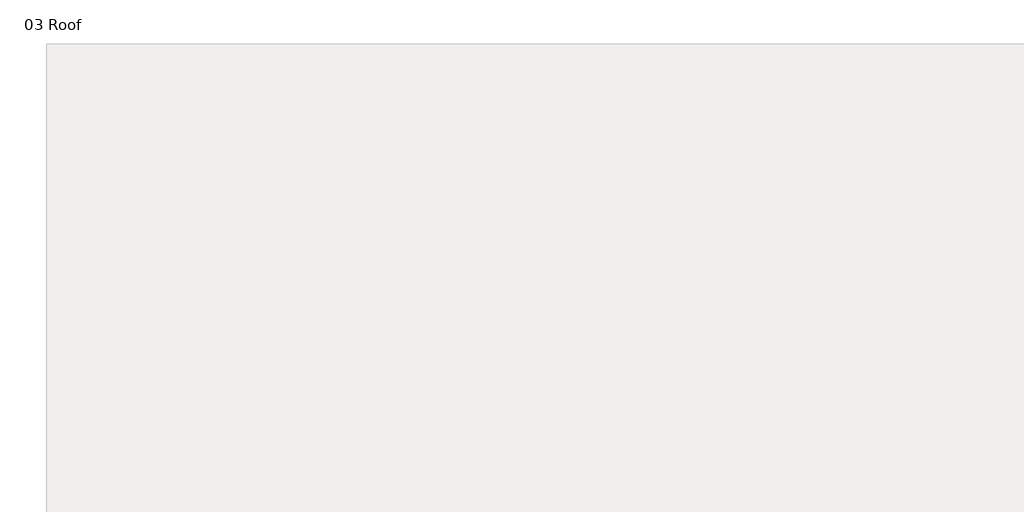
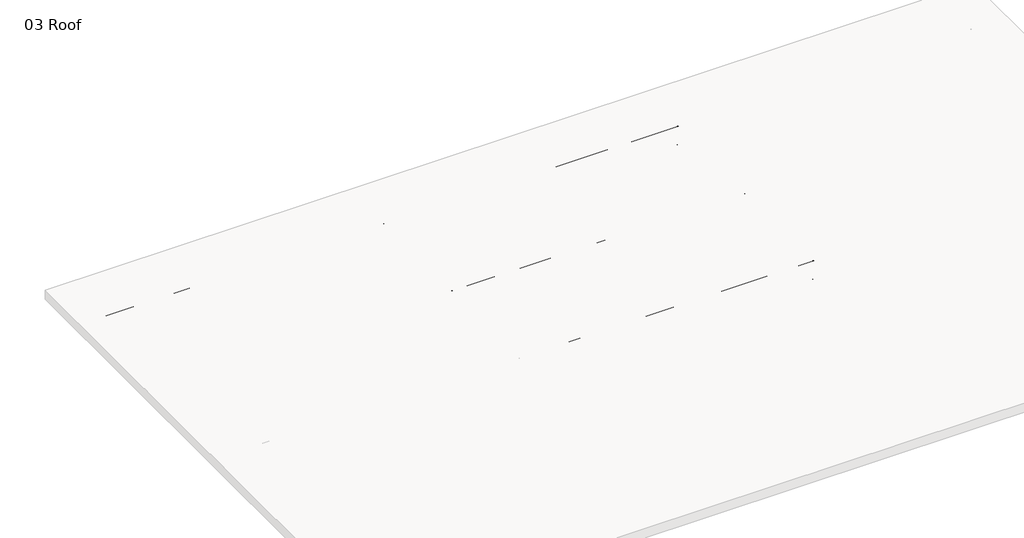
# One storey, part 3 of 4: 102 beams.
"""IFC4 building model written with IfcOpenShell, lengths in millimetres."""

import ifcopenshell
import ifcopenshell.guid

model = None  # the IFC model being written
_history = None  # IfcOwnerHistory: only IFC2X3 demands one
_inside = {}  # id of a spatial element -> (the spatial element, [elements in it])
_under = {}  # id of a project, library or spatial element -> (it, [spatial elements below it])
_declared = {}  # id of a project -> (the project, [libraries it declares])
_typed = {}  # id of a type object -> (the type object, [elements of that type])
_made_of = {}  # id of a material, layer set ... -> (it, [elements and type objects made of it])


def new_model(schema):
    """Start an empty IFC model of exactly this schema.

    Asked for "IFC4X3", IfcOpenShell would pick the latest addendum, in which some entities
    have other attributes; the version numbers below select the first issue.
    IFC2X3 requires an IfcOwnerHistory on every rooted entity: one is made here for all.
    """
    global model, _history
    if schema == "IFC4X3":
        model = ifcopenshell.file(schema_version=(4, 3, 0, 0))
    else:
        model = ifcopenshell.file(schema=schema)
    _inside.clear()
    _under.clear()
    _declared.clear()
    _typed.clear()
    _made_of.clear()
    _history = None
    if model.schema == "IFC2X3":
        org = make("IfcOrganization", Name="unknown")
        user = make(
            "IfcPersonAndOrganization",
            ThePerson=make("IfcPerson", FamilyName="unknown"),
            TheOrganization=org,
        )
        app = make(
            "IfcApplication",
            ApplicationDeveloper=org,
            Version="unknown",
            ApplicationFullName="unknown",
            ApplicationIdentifier="unknown",
        )
        _history = make(
            "IfcOwnerHistory",
            OwningUser=user,
            OwningApplication=app,
            ChangeAction="ADDED",
            CreationDate=0,
        )
    return model


def make(cls, **values):
    """One entity of the class cls with the attributes given. An attribute that is None is left unset."""
    return model.create_entity(
        cls, **{name: value for name, value in values.items() if value is not None}
    )


def rooted(cls, **values):
    """An entity with a GlobalId (a new one), such as an element, a storey or a relation."""
    return make(cls, GlobalId=ifcopenshell.guid.new(), OwnerHistory=_history, **values)


def si_unit(unit_type, name, prefix=None):
    """IfcSIUnit, for example si_unit("LENGTHUNIT", "METRE", prefix="MILLI")."""
    return make("IfcSIUnit", UnitType=unit_type, Prefix=prefix, Name=name)


def assignment(units):
    """IfcUnitAssignment: the units of a project."""
    return None if units is None else make("IfcUnitAssignment", Units=units)


def point(xyz):
    """IfcCartesianPoint."""
    return None if xyz is None else make("IfcCartesianPoint", Coordinates=xyz)


def direction(xyz):
    """IfcDirection."""
    return None if xyz is None else make("IfcDirection", DirectionRatios=xyz)


def frame(location, z_axis=None, x_axis=None):
    """IfcAxis2Placement3D, a coordinate frame: its origin and axes. An axis left out is left unset."""
    return make(
        "IfcAxis2Placement3D",
        Location=point(location),
        Axis=direction(z_axis),
        RefDirection=direction(x_axis),
    )


def frame_2d(location, x_axis=None):
    """IfcAxis2Placement2D, a coordinate frame in the plane: its origin and x axis."""
    return make(
        "IfcAxis2Placement2D", Location=point(location), RefDirection=direction(x_axis)
    )


def origin():
    """The frame at (0, 0, 0) with its axes left unset."""
    return frame((0.0, 0.0, 0.0))


def place(relative_to, where):
    """IfcLocalPlacement: puts the frame where relative to a parent placement (None: the world)."""
    return make(
        "IfcLocalPlacement", PlacementRelTo=relative_to, RelativePlacement=where
    )


def context(
    kind, dimensions, precision=None, world=None, true_north=None, identifier=None
):
    """IfcGeometricRepresentationContext, for example the 3D "Model" context."""
    return make(
        "IfcGeometricRepresentationContext",
        ContextIdentifier=identifier,
        ContextType=kind,
        CoordinateSpaceDimension=dimensions,
        Precision=precision,
        WorldCoordinateSystem=world,
        TrueNorth=true_north,
    )


def project(units=None, contexts=None):
    """IfcProject with its units and contexts."""
    return rooted(
        "IfcProject",
        Name="project",
        RepresentationContexts=contexts,
        UnitsInContext=assignment(units),
    )


def spatial(cls, under=None, at=None, **own):
    """A site, building, storey or space (cls), placed at a placement, below another one or the project."""
    s = rooted(cls, ObjectPlacement=at, **own)
    if under is not None:
        _under.setdefault(under.id(), (under, []))[1].append(s)
    return s


def polyline(points):
    """IfcPolyline through the points."""
    return make("IfcPolyline", Points=[point(p) for p in points])


def circle_curve(where, radius):
    """IfcCircle in the frame where."""
    return make("IfcCircle", Position=where, Radius=radius)


def trimmed(basis, trim1, trim2, sense, master):
    """IfcTrimmedCurve: the piece of a basis curve between two trims."""
    return make(
        "IfcTrimmedCurve",
        BasisCurve=basis,
        Trim1=trim1,
        Trim2=trim2,
        SenseAgreement=sense,
        MasterRepresentation=master,
    )


def segment(curve, same_sense, transition):
    """IfcCompositeCurveSegment."""
    return make(
        "IfcCompositeCurveSegment",
        Transition=transition,
        SameSense=same_sense,
        ParentCurve=curve,
    )


def composite_curve(segments, self_intersect=None):
    """IfcCompositeCurve: segments joined end to end."""
    return make("IfcCompositeCurve", Segments=segments, SelfIntersect=self_intersect)


def outline(outer, holes=None, kind="AREA"):
    """IfcArbitraryClosedProfileDef: a profile drawn as a closed curve; with holes, ...WithVoids."""
    if holes is None:
        return make("IfcArbitraryClosedProfileDef", ProfileType=kind, OuterCurve=outer)
    return make(
        "IfcArbitraryProfileDefWithVoids",
        ProfileType=kind,
        OuterCurve=outer,
        InnerCurves=holes,
    )


def extrude(swept, where, along, depth):
    """IfcExtrudedAreaSolid: the profile swept, set in the frame where, extruded along a direction by depth."""
    return make(
        "IfcExtrudedAreaSolid",
        SweptArea=swept,
        Position=where,
        ExtrudedDirection=direction(along),
        Depth=depth,
    )


def shape(context_of_items, identifier, shape_type, items):
    """IfcShapeRepresentation: the items that make up one representation, for example the "Body"."""
    return make(
        "IfcShapeRepresentation",
        ContextOfItems=context_of_items,
        RepresentationIdentifier=identifier,
        RepresentationType=shape_type,
        Items=items,
    )


def source(mapping_origin, context_of_items, identifier, shape_type, items):
    """IfcRepresentationMap: a shape defined once, which mapped items show again and again."""
    return make(
        "IfcRepresentationMap",
        MappingOrigin=mapping_origin,
        MappedRepresentation=shape(context_of_items, identifier, shape_type, items),
    )


def transform(
    local_origin,
    x_axis=None,
    y_axis=None,
    z_axis=None,
    scale=None,
    scale2=None,
    scale3=None,
    uniform=True,
):
    """IfcCartesianTransformationOperator3D, or its non-uniform kind. x_axis, y_axis, z_axis: its Axis1, 2, 3."""
    if uniform:
        return make(
            "IfcCartesianTransformationOperator3D",
            Axis1=direction(x_axis),
            Axis2=direction(y_axis),
            LocalOrigin=point(local_origin),
            Scale=scale,
            Axis3=direction(z_axis),
        )
    return make(
        "IfcCartesianTransformationOperator3DnonUniform",
        Axis1=direction(x_axis),
        Axis2=direction(y_axis),
        LocalOrigin=point(local_origin),
        Scale=scale,
        Axis3=direction(z_axis),
        Scale2=scale2,
        Scale3=scale3,
    )


def mapped(mapping_source, mapping_target):
    """IfcMappedItem: shows the shape of a source again, moved by a transform."""
    return make(
        "IfcMappedItem", MappingSource=mapping_source, MappingTarget=mapping_target
    )


def made_of(thing, what):
    """Note that an element or type object is made of a material, layer set ...; save() writes the relation."""
    if what is not None:
        _made_of.setdefault(what.id(), (what, []))[1].append(thing)
    return thing


def element(
    cls,
    number,
    at=None,
    inside=None,
    cuts=None,
    type_object=None,
    material=None,
    context=None,
    identifier="Body",
    shape_type=None,
    held_by="IfcProductDefinitionShape",
    body=None,
    shapes=None,
    **own,
):
    """One element of the class cls, such as IfcWall. Its Tag is "e" and its number.

    at: its placement. inside: the storey or other place that contains it. cuts: it is an
    opening in that element (IfcRelVoidsElement). A single representation is given by context,
    identifier, shape_type and body (its items); several are given by shapes. held_by: the class
    of the entity that holds the representations. save() writes the other relations.
    """
    e = rooted(cls, Tag="e%d" % number, ObjectPlacement=at, **own)
    if body is not None:
        shapes = [shape(context, identifier, shape_type, body)]
    if shapes is not None:
        e.Representation = make(held_by, Representations=shapes)
    if inside is not None:
        _inside.setdefault(inside.id(), (inside, []))[1].append(e)
    if cuts is not None:
        rooted(
            "IfcRelVoidsElement", RelatingBuildingElement=cuts, RelatedOpeningElement=e
        )
    if type_object is not None:
        _typed.setdefault(type_object.id(), (type_object, []))[1].append(e)
    return made_of(e, material)


def aggregate(whole, parts):
    """IfcRelAggregates: a whole, such as a stair, and the parts it consists of."""
    return rooted("IfcRelAggregates", RelatingObject=whole, RelatedObjects=parts)


def save(model, path):
    """Write the relations noted so far, then the file.

    IfcRelAggregates (storeys below a building ...), IfcRelContainedInSpatialStructure (elements
    in a storey), IfcRelDefinesByType, IfcRelAssociatesMaterial and IfcRelDeclares: one each for
    every whole, place, type object, material and project.
    """
    for whole, parts in _under.values():
        aggregate(whole, parts)
    for where, things in _inside.values():
        rooted(
            "IfcRelContainedInSpatialStructure",
            RelatedElements=things,
            RelatingStructure=where,
        )
    for kind, things in _typed.values():
        rooted("IfcRelDefinesByType", RelatedObjects=things, RelatingType=kind)
    for what, things in _made_of.values():
        rooted("IfcRelAssociatesMaterial", RelatedObjects=things, RelatingMaterial=what)
    for by, libraries in _declared.values():
        rooted("IfcRelDeclares", RelatingContext=by, RelatedDefinitions=libraries)
    model.write(path)


def ub_universal_beam_305x165x40ub_24de31be(model_context):
    return source(origin(), model_context, "Body", "SweptSolid", [
        extrude(outline(composite_curve([segment(polyline([(82.5, -141.5), (82.5, -151.7), (-82.5, -151.7), (-82.5, -141.5), (-11.9, -141.5)]), True, "CONTINUOUS"), segment(trimmed(circle_curve(frame_2d((-11.9, -132.6)), 8.9), [point((-11.9, -141.5))], [point((-3.0, -132.6))], True, "CARTESIAN"), True, "CONTINUOUS"), segment(polyline([(-3.0, -132.6), (-3.0, 132.6)]), True, "CONTINUOUS"), segment(trimmed(circle_curve(frame_2d((-11.9, 132.6)), 8.9), [point((-3.0, 132.6))], [point((-11.9, 141.5))], True, "CARTESIAN"), True, "CONTINUOUS"), segment(polyline([(-11.9, 141.5), (-82.5, 141.5), (-82.5, 151.7), (82.5, 151.7), (82.5, 141.5), (11.9, 141.5)]), True, "CONTINUOUS"), segment(trimmed(circle_curve(frame_2d((11.9, 132.6)), 8.9), [point((11.9, 141.5))], [point((3.0, 132.6))], True, "CARTESIAN"), True, "CONTINUOUS"), segment(polyline([(3.0, 132.6), (3.0, -132.6)]), True, "CONTINUOUS"), segment(trimmed(circle_curve(frame_2d((11.9, -132.6)), 8.9), [point((3.0, -132.6))], [point((11.9, -141.5))], True, "CARTESIAN"), True, "CONTINUOUS"), segment(polyline([(11.9, -141.5), (82.5, -141.5)]), True, "CONTINUOUS")], self_intersect=False)), frame((-335.6, 0.0, 0.0), z_axis=(1.0, 0.0, 0.0), x_axis=(0.0, 1.0, 0.0)), (0.0, 0.0, 1.0), 671.2),
    ])


def ub_universal_beam_305x165x40ub_f67fc52f(model_context):
    return source(origin(), model_context, "Body", "SweptSolid", [
        extrude(outline(composite_curve([segment(polyline([(82.5, -141.5), (82.5, -151.7), (-82.5, -151.7), (-82.5, -141.5), (-11.9, -141.5)]), True, "CONTINUOUS"), segment(trimmed(circle_curve(frame_2d((-11.9, -132.6)), 8.9), [point((-11.9, -141.5))], [point((-3.0, -132.6))], True, "CARTESIAN"), True, "CONTINUOUS"), segment(polyline([(-3.0, -132.6), (-3.0, 132.6)]), True, "CONTINUOUS"), segment(trimmed(circle_curve(frame_2d((-11.9, 132.6)), 8.9), [point((-3.0, 132.6))], [point((-11.9, 141.5))], True, "CARTESIAN"), True, "CONTINUOUS"), segment(polyline([(-11.9, 141.5), (-82.5, 141.5), (-82.5, 151.7), (82.5, 151.7), (82.5, 141.5), (11.9, 141.5)]), True, "CONTINUOUS"), segment(trimmed(circle_curve(frame_2d((11.9, 132.6)), 8.9), [point((11.9, 141.5))], [point((3.0, 132.6))], True, "CARTESIAN"), True, "CONTINUOUS"), segment(polyline([(3.0, 132.6), (3.0, -132.6)]), True, "CONTINUOUS"), segment(trimmed(circle_curve(frame_2d((11.9, -132.6)), 8.9), [point((3.0, -132.6))], [point((11.9, -141.5))], True, "CARTESIAN"), True, "CONTINUOUS"), segment(polyline([(11.9, -141.5), (82.5, -141.5)]), True, "CONTINUOUS")], self_intersect=False)), frame((-7125.0, 0.0, 0.0), z_axis=(1.0, 0.0, 0.0), x_axis=(0.0, 1.0, 0.0)), (0.0, 0.0, 1.0), 14250.0),
    ])


def ub_universal_beam_305x165x40ub_26fb8d3a(model_context):
    return source(origin(), model_context, "Body", "SweptSolid", [
        extrude(outline(composite_curve([segment(polyline([(82.5, -141.5), (82.5, -151.7), (-82.5, -151.7), (-82.5, -141.5), (-11.9, -141.5)]), True, "CONTINUOUS"), segment(trimmed(circle_curve(frame_2d((-11.9, -132.6)), 8.9), [point((-11.9, -141.5))], [point((-3.0, -132.6))], True, "CARTESIAN"), True, "CONTINUOUS"), segment(polyline([(-3.0, -132.6), (-3.0, 132.6)]), True, "CONTINUOUS"), segment(trimmed(circle_curve(frame_2d((-11.9, 132.6)), 8.9), [point((-3.0, 132.6))], [point((-11.9, 141.5))], True, "CARTESIAN"), True, "CONTINUOUS"), segment(polyline([(-11.9, 141.5), (-82.5, 141.5), (-82.5, 151.7), (82.5, 151.7), (82.5, 141.5), (11.9, 141.5)]), True, "CONTINUOUS"), segment(trimmed(circle_curve(frame_2d((11.9, 132.6)), 8.9), [point((11.9, 141.5))], [point((3.0, 132.6))], True, "CARTESIAN"), True, "CONTINUOUS"), segment(polyline([(3.0, 132.6), (3.0, -132.6)]), True, "CONTINUOUS"), segment(trimmed(circle_curve(frame_2d((11.9, -132.6)), 8.9), [point((3.0, -132.6))], [point((11.9, -141.5))], True, "CARTESIAN"), True, "CONTINUOUS"), segment(polyline([(11.9, -141.5), (82.5, -141.5)]), True, "CONTINUOUS")], self_intersect=False)), frame((-347.8807825, 0.0, 0.0), z_axis=(1.0, 0.0, 0.0), x_axis=(0.0, 1.0, 0.0)), (0.0, 0.0, 1.0), 695.761565),
    ])


model = new_model("IFC4")

# Units and contexts
model_context = context("Model", 3, world=origin())
ifc_project = project(units=[si_unit("LENGTHUNIT", "METRE", prefix="MILLI")], contexts=[model_context])

# Site, building, storey
site = spatial("IfcSite", under=ifc_project)
building = spatial("IfcBuilding", under=site)
storey = spatial("IfcBuildingStorey", under=building, Name="03 Roof", Elevation=8000.0)

# Beams
placement = place(None, origin())
ub_universal_beam_305x165x40ub_shape = ub_universal_beam_305x165x40ub_24de31be(model_context)
element("IfcBeam", 1, ObjectType="UB-Universal Beam : 305x165x40UB", at=placement, inside=storey, context=model_context, shape_type="MappedRepresentation", body=[
    mapped(ub_universal_beam_305x165x40ub_shape, transform((-9276.5506826, 12261.9474871, 7500.0), x_axis=(0.0, 0.0, 1.0), y_axis=(0.0, -1.0, 0.0), z_axis=(1.0, 0.0, 0.0))),
])
element("IfcBeam", 2, ObjectType="UB-Universal Beam : 305x165x40UB", at=placement, inside=storey, context=model_context, shape_type="MappedRepresentation", body=[
    mapped(ub_universal_beam_305x165x40ub_shape, transform((-10464.0506826, 12261.9474871, 7500.0), x_axis=(0.0, 0.0, 1.0), y_axis=(0.0, -1.0, 0.0), z_axis=(1.0, 0.0, 0.0))),
])
element("IfcBeam", 3, ObjectType="UB-Universal Beam : 305x165x40UB", at=placement, inside=storey, context=model_context, shape_type="MappedRepresentation", body=[
    mapped(ub_universal_beam_305x165x40ub_shape, transform((-11651.5506826, 12261.9474871, 7500.0), x_axis=(0.0, 0.0, 1.0), y_axis=(0.0, -1.0, 0.0), z_axis=(1.0, 0.0, 0.0))),
])
element("IfcBeam", 4, ObjectType="UB-Universal Beam : 305x165x40UB", at=placement, inside=storey, context=model_context, shape_type="MappedRepresentation", body=[
    mapped(ub_universal_beam_305x165x40ub_shape, transform((-12839.0506826, 12261.9474871, 7500.0), x_axis=(0.0, 0.0, 1.0), y_axis=(0.0, -1.0, 0.0), z_axis=(1.0, 0.0, 0.0))),
])
element("IfcBeam", 5, ObjectType="UB-Universal Beam : 305x165x40UB", at=placement, inside=storey, context=model_context, shape_type="MappedRepresentation", body=[
    mapped(ub_universal_beam_305x165x40ub_shape, transform((-8089.0506826, 12261.9474871, 7500.0), x_axis=(0.0, 0.0, 1.0), y_axis=(0.0, -1.0, 0.0), z_axis=(1.0, 0.0, 0.0))),
])
element("IfcBeam", 6, ObjectType="UB-Universal Beam : 305x165x40UB", at=placement, inside=storey, context=model_context, shape_type="MappedRepresentation", body=[
    mapped(ub_universal_beam_305x165x40ub_shape, transform((-14026.5506826, 12261.9474871, 7500.0), x_axis=(0.0, 0.0, 1.0), y_axis=(0.0, -1.0, 0.0), z_axis=(1.0, 0.0, 0.0))),
])
element("IfcBeam", 7, ObjectType="UB-Universal Beam : 305x165x40UB", at=placement, inside=storey, context=model_context, shape_type="MappedRepresentation", body=[
    mapped(ub_universal_beam_305x165x40ub_shape, transform((-15214.0506826, 12261.9474871, 7500.0), x_axis=(0.0, 0.0, 1.0), y_axis=(0.0, -1.0, 0.0), z_axis=(1.0, 0.0, 0.0))),
])
element("IfcBeam", 8, ObjectType="UB-Universal Beam : 305x165x40UB", at=placement, inside=storey, context=model_context, shape_type="MappedRepresentation", body=[
    mapped(ub_universal_beam_305x165x40ub_shape, transform((-6151.5506826, 12261.9474871, 7500.0), x_axis=(0.0, 0.0, 1.0), y_axis=(0.0, -1.0, 0.0), z_axis=(1.0, 0.0, 0.0))),
])
element("IfcBeam", 9, ObjectType="UB-Universal Beam : 305x165x40UB", at=placement, inside=storey, context=model_context, shape_type="MappedRepresentation", body=[
    mapped(ub_universal_beam_305x165x40ub_shape, transform((-4964.0506826, 12261.9474871, 7500.0), x_axis=(0.0, 0.0, 1.0), y_axis=(0.0, -1.0, 0.0), z_axis=(1.0, 0.0, 0.0))),
])
element("IfcBeam", 10, ObjectType="UB-Universal Beam : 305x165x40UB", at=placement, inside=storey, context=model_context, shape_type="MappedRepresentation", body=[
    mapped(ub_universal_beam_305x165x40ub_shape, transform((-3776.5506826, 12261.9474871, 7500.0), x_axis=(0.0, 0.0, 1.0), y_axis=(0.0, -1.0, 0.0), z_axis=(1.0, 0.0, 0.0))),
])
element("IfcBeam", 11, ObjectType="UB-Universal Beam : 305x165x40UB", at=placement, inside=storey, context=model_context, shape_type="MappedRepresentation", body=[
    mapped(ub_universal_beam_305x165x40ub_shape, transform((-2589.0506826, 12261.9474871, 7500.0), x_axis=(0.0, 0.0, 1.0), y_axis=(0.0, -1.0, 0.0), z_axis=(1.0, 0.0, 0.0))),
])
element("IfcBeam", 12, ObjectType="UB-Universal Beam : 305x165x40UB", at=placement, inside=storey, context=model_context, shape_type="MappedRepresentation", body=[
    mapped(ub_universal_beam_305x165x40ub_shape, transform((-7339.0506826, 12261.9474871, 7500.0), x_axis=(0.0, 0.0, 1.0), y_axis=(0.0, -1.0, 0.0), z_axis=(1.0, 0.0, 0.0))),
])
element("IfcBeam", 13, ObjectType="UB-Universal Beam : 305x165x40UB", at=placement, inside=storey, context=model_context, shape_type="MappedRepresentation", body=[
    mapped(ub_universal_beam_305x165x40ub_shape, transform((-1401.5506826, 12261.9474871, 7500.0), x_axis=(0.0, 0.0, 1.0), y_axis=(0.0, -1.0, 0.0), z_axis=(1.0, 0.0, 0.0))),
])
element("IfcBeam", 14, ObjectType="UB-Universal Beam : 305x165x40UB", at=placement, inside=storey, context=model_context, shape_type="MappedRepresentation", body=[
    mapped(ub_universal_beam_305x165x40ub_shape, transform((-214.0506826, 12261.9474871, 7500.0), x_axis=(0.0, 0.0, 1.0), y_axis=(0.0, -1.0, 0.0), z_axis=(1.0, 0.0, 0.0))),
])
element("IfcBeam", 15, ObjectType="UB-Universal Beam : 305x165x40UB", at=placement, inside=storey, context=model_context, shape_type="MappedRepresentation", body=[
    mapped(ub_universal_beam_305x165x40ub_shape, transform((-9276.5506826, 6271.8474871, 7500.0), x_axis=(0.0, 0.0, 1.0), y_axis=(0.0, -1.0, 0.0), z_axis=(1.0, 0.0, 0.0))),
])
element("IfcBeam", 16, ObjectType="UB-Universal Beam : 305x165x40UB", at=placement, inside=storey, context=model_context, shape_type="MappedRepresentation", body=[
    mapped(ub_universal_beam_305x165x40ub_shape, transform((-10464.0506826, 6271.8474871, 7500.0), x_axis=(0.0, 0.0, 1.0), y_axis=(0.0, -1.0, 0.0), z_axis=(1.0, 0.0, 0.0))),
])
element("IfcBeam", 17, ObjectType="UB-Universal Beam : 305x165x40UB", at=placement, inside=storey, context=model_context, shape_type="MappedRepresentation", body=[
    mapped(ub_universal_beam_305x165x40ub_shape, transform((-11651.5506826, 6271.8474871, 7500.0), x_axis=(0.0, 0.0, 1.0), y_axis=(0.0, -1.0, 0.0), z_axis=(1.0, 0.0, 0.0))),
])
element("IfcBeam", 18, ObjectType="UB-Universal Beam : 305x165x40UB", at=placement, inside=storey, context=model_context, shape_type="MappedRepresentation", body=[
    mapped(ub_universal_beam_305x165x40ub_shape, transform((-12839.0506826, 6271.8474871, 7500.0), x_axis=(0.0, 0.0, 1.0), y_axis=(0.0, -1.0, 0.0), z_axis=(1.0, 0.0, 0.0))),
])
element("IfcBeam", 19, ObjectType="UB-Universal Beam : 305x165x40UB", at=placement, inside=storey, context=model_context, shape_type="MappedRepresentation", body=[
    mapped(ub_universal_beam_305x165x40ub_shape, transform((-8089.0506826, 6271.8474871, 7500.0), x_axis=(0.0, 0.0, 1.0), y_axis=(0.0, -1.0, 0.0), z_axis=(1.0, 0.0, 0.0))),
])
element("IfcBeam", 20, ObjectType="UB-Universal Beam : 305x165x40UB", at=placement, inside=storey, context=model_context, shape_type="MappedRepresentation", body=[
    mapped(ub_universal_beam_305x165x40ub_shape, transform((-14026.5506826, 6271.8474871, 7500.0), x_axis=(0.0, 0.0, 1.0), y_axis=(0.0, -1.0, 0.0), z_axis=(1.0, 0.0, 0.0))),
])
element("IfcBeam", 21, ObjectType="UB-Universal Beam : 305x165x40UB", at=placement, inside=storey, context=model_context, shape_type="MappedRepresentation", body=[
    mapped(ub_universal_beam_305x165x40ub_shape, transform((-15214.0506826, 6271.8474871, 7500.0), x_axis=(0.0, 0.0, 1.0), y_axis=(0.0, -1.0, 0.0), z_axis=(1.0, 0.0, 0.0))),
])
element("IfcBeam", 22, ObjectType="UB-Universal Beam : 305x165x40UB", at=placement, inside=storey, context=model_context, shape_type="MappedRepresentation", body=[
    mapped(ub_universal_beam_305x165x40ub_shape, transform((-6151.5506826, 6271.8474871, 7500.0), x_axis=(0.0, 0.0, 1.0), y_axis=(0.0, -1.0, 0.0), z_axis=(1.0, 0.0, 0.0))),
])
element("IfcBeam", 23, ObjectType="UB-Universal Beam : 305x165x40UB", at=placement, inside=storey, context=model_context, shape_type="MappedRepresentation", body=[
    mapped(ub_universal_beam_305x165x40ub_shape, transform((-4964.0506826, 6271.8474871, 7500.0), x_axis=(0.0, 0.0, 1.0), y_axis=(0.0, -1.0, 0.0), z_axis=(1.0, 0.0, 0.0))),
])
element("IfcBeam", 24, ObjectType="UB-Universal Beam : 305x165x40UB", at=placement, inside=storey, context=model_context, shape_type="MappedRepresentation", body=[
    mapped(ub_universal_beam_305x165x40ub_shape, transform((973.4493174, 6271.8474871, 7500.0), x_axis=(0.0, 0.0, 1.0), y_axis=(0.0, -1.0, 0.0), z_axis=(1.0, 0.0, 0.0))),
])
element("IfcBeam", 25, ObjectType="UB-Universal Beam : 305x165x40UB", at=placement, inside=storey, context=model_context, shape_type="MappedRepresentation", body=[
    mapped(ub_universal_beam_305x165x40ub_shape, transform((-3776.5506826, 6271.8474871, 7500.0), x_axis=(0.0, 0.0, 1.0), y_axis=(0.0, -1.0, 0.0), z_axis=(1.0, 0.0, 0.0))),
])
element("IfcBeam", 26, ObjectType="UB-Universal Beam : 305x165x40UB", at=placement, inside=storey, context=model_context, shape_type="MappedRepresentation", body=[
    mapped(ub_universal_beam_305x165x40ub_shape, transform((-2589.0506826, 6271.8474871, 7500.0), x_axis=(0.0, 0.0, 1.0), y_axis=(0.0, -1.0, 0.0), z_axis=(1.0, 0.0, 0.0))),
])
element("IfcBeam", 27, ObjectType="UB-Universal Beam : 305x165x40UB", at=placement, inside=storey, context=model_context, shape_type="MappedRepresentation", body=[
    mapped(ub_universal_beam_305x165x40ub_shape, transform((-7339.0506826, 6271.8474871, 7500.0), x_axis=(0.0, 0.0, 1.0), y_axis=(0.0, -1.0, 0.0), z_axis=(1.0, 0.0, 0.0))),
])
element("IfcBeam", 28, ObjectType="UB-Universal Beam : 305x165x40UB", at=placement, inside=storey, context=model_context, shape_type="MappedRepresentation", body=[
    mapped(ub_universal_beam_305x165x40ub_shape, transform((-1401.5506826, 6271.8474871, 7500.0), x_axis=(0.0, 0.0, 1.0), y_axis=(0.0, -1.0, 0.0), z_axis=(1.0, 0.0, 0.0))),
])
element("IfcBeam", 29, ObjectType="UB-Universal Beam : 305x165x40UB", at=placement, inside=storey, context=model_context, shape_type="MappedRepresentation", body=[
    mapped(ub_universal_beam_305x165x40ub_shape, transform((-214.0506826, 6271.8474871, 7500.0), x_axis=(0.0, 0.0, 1.0), y_axis=(0.0, -1.0, 0.0), z_axis=(1.0, 0.0, 0.0))),
])
element("IfcBeam", 30, ObjectType="UB-Universal Beam : 305x165x40UB", at=placement, inside=storey, context=model_context, shape_type="MappedRepresentation", body=[
    mapped(ub_universal_beam_305x165x40ub_shape, transform((7660.9493174, 271.8474871, 7500.0), x_axis=(0.0, 0.0, 1.0), y_axis=(0.0, -1.0, 0.0), z_axis=(1.0, 0.0, 0.0))),
])
element("IfcBeam", 31, ObjectType="UB-Universal Beam : 305x165x40UB", at=placement, inside=storey, context=model_context, shape_type="MappedRepresentation", body=[
    mapped(ub_universal_beam_305x165x40ub_shape, transform((5723.4493174, 271.8474871, 7500.0), x_axis=(0.0, 0.0, 1.0), y_axis=(0.0, -1.0, 0.0), z_axis=(1.0, 0.0, 0.0))),
])
element("IfcBeam", 32, ObjectType="UB-Universal Beam : 305x165x40UB", at=placement, inside=storey, context=model_context, shape_type="MappedRepresentation", body=[
    mapped(ub_universal_beam_305x165x40ub_shape, transform((-6151.5506826, 271.8474871, 7500.0), x_axis=(0.0, 0.0, 1.0), y_axis=(0.0, -1.0, 0.0), z_axis=(1.0, 0.0, 0.0))),
])
element("IfcBeam", 33, ObjectType="UB-Universal Beam : 305x165x40UB", at=placement, inside=storey, context=model_context, shape_type="MappedRepresentation", body=[
    mapped(ub_universal_beam_305x165x40ub_shape, transform((4535.9493174, 271.8474871, 7500.0), x_axis=(0.0, 0.0, 1.0), y_axis=(0.0, -1.0, 0.0), z_axis=(1.0, 0.0, 0.0))),
])
element("IfcBeam", 34, ObjectType="UB-Universal Beam : 305x165x40UB", at=placement, inside=storey, context=model_context, shape_type="MappedRepresentation", body=[
    mapped(ub_universal_beam_305x165x40ub_shape, transform((-4964.0506826, 271.8474871, 7500.0), x_axis=(0.0, 0.0, 1.0), y_axis=(0.0, -1.0, 0.0), z_axis=(1.0, 0.0, 0.0))),
])
element("IfcBeam", 35, ObjectType="UB-Universal Beam : 305x165x40UB", at=placement, inside=storey, context=model_context, shape_type="MappedRepresentation", body=[
    mapped(ub_universal_beam_305x165x40ub_shape, transform((3348.4493174, 271.8474871, 7500.0), x_axis=(0.0, 0.0, 1.0), y_axis=(0.0, -1.0, 0.0), z_axis=(1.0, 0.0, 0.0))),
])
element("IfcBeam", 36, ObjectType="UB-Universal Beam : 305x165x40UB", at=placement, inside=storey, context=model_context, shape_type="MappedRepresentation", body=[
    mapped(ub_universal_beam_305x165x40ub_shape, transform((2160.9493174, 271.8474871, 7500.0), x_axis=(0.0, 0.0, 1.0), y_axis=(0.0, -1.0, 0.0), z_axis=(1.0, 0.0, 0.0))),
])
element("IfcBeam", 37, ObjectType="UB-Universal Beam : 305x165x40UB", at=placement, inside=storey, context=model_context, shape_type="MappedRepresentation", body=[
    mapped(ub_universal_beam_305x165x40ub_shape, transform((6910.9493174, 271.8474871, 7500.0), x_axis=(0.0, 0.0, 1.0), y_axis=(0.0, -1.0, 0.0), z_axis=(1.0, 0.0, 0.0))),
])
element("IfcBeam", 38, ObjectType="UB-Universal Beam : 305x165x40UB", at=placement, inside=storey, context=model_context, shape_type="MappedRepresentation", body=[
    mapped(ub_universal_beam_305x165x40ub_shape, transform((973.4493174, 271.8474871, 7500.0), x_axis=(0.0, 0.0, 1.0), y_axis=(0.0, -1.0, 0.0), z_axis=(1.0, 0.0, 0.0))),
])
element("IfcBeam", 39, ObjectType="UB-Universal Beam : 305x165x40UB", at=placement, inside=storey, context=model_context, shape_type="MappedRepresentation", body=[
    mapped(ub_universal_beam_305x165x40ub_shape, transform((-3776.5506826, 271.8474871, 7500.0), x_axis=(0.0, 0.0, 1.0), y_axis=(0.0, -1.0, 0.0), z_axis=(1.0, 0.0, 0.0))),
])
element("IfcBeam", 40, ObjectType="UB-Universal Beam : 305x165x40UB", at=placement, inside=storey, context=model_context, shape_type="MappedRepresentation", body=[
    mapped(ub_universal_beam_305x165x40ub_shape, transform((-2589.0506826, 271.8474871, 7500.0), x_axis=(0.0, 0.0, 1.0), y_axis=(0.0, -1.0, 0.0), z_axis=(1.0, 0.0, 0.0))),
])
element("IfcBeam", 41, ObjectType="UB-Universal Beam : 305x165x40UB", at=placement, inside=storey, context=model_context, shape_type="MappedRepresentation", body=[
    mapped(ub_universal_beam_305x165x40ub_shape, transform((-7339.0506826, 271.8474871, 7500.0), x_axis=(0.0, 0.0, 1.0), y_axis=(0.0, -1.0, 0.0), z_axis=(1.0, 0.0, 0.0))),
])
element("IfcBeam", 42, ObjectType="UB-Universal Beam : 305x165x40UB", at=placement, inside=storey, context=model_context, shape_type="MappedRepresentation", body=[
    mapped(ub_universal_beam_305x165x40ub_shape, transform((-1401.5506826, 271.8474871, 7500.0), x_axis=(0.0, 0.0, 1.0), y_axis=(0.0, -1.0, 0.0), z_axis=(1.0, 0.0, 0.0))),
])
element("IfcBeam", 43, ObjectType="UB-Universal Beam : 305x165x40UB", at=placement, inside=storey, context=model_context, shape_type="MappedRepresentation", body=[
    mapped(ub_universal_beam_305x165x40ub_shape, transform((-214.0506826, 271.8474871, 7500.0), x_axis=(0.0, 0.0, 1.0), y_axis=(0.0, -1.0, 0.0), z_axis=(1.0, 0.0, 0.0))),
])
element("IfcBeam", 44, ObjectType="UB-Universal Beam : 305x165x40UB", at=placement, inside=storey, context=model_context, shape_type="MappedRepresentation", body=[
    mapped(ub_universal_beam_305x165x40ub_shape, transform((-9276.5506826, 271.8474871, 7500.0), x_axis=(0.0, 0.0, 1.0), y_axis=(0.0, -1.0, 0.0), z_axis=(1.0, 0.0, 0.0))),
])
element("IfcBeam", 45, ObjectType="UB-Universal Beam : 305x165x40UB", at=placement, inside=storey, context=model_context, shape_type="MappedRepresentation", body=[
    mapped(ub_universal_beam_305x165x40ub_shape, transform((-10464.0506826, 271.8474871, 7500.0), x_axis=(0.0, 0.0, 1.0), y_axis=(0.0, -1.0, 0.0), z_axis=(1.0, 0.0, 0.0))),
])
element("IfcBeam", 46, ObjectType="UB-Universal Beam : 305x165x40UB", at=placement, inside=storey, context=model_context, shape_type="MappedRepresentation", body=[
    mapped(ub_universal_beam_305x165x40ub_shape, transform((-11651.5506826, 271.8474871, 7500.0), x_axis=(0.0, 0.0, 1.0), y_axis=(0.0, -1.0, 0.0), z_axis=(1.0, 0.0, 0.0))),
])
element("IfcBeam", 47, ObjectType="UB-Universal Beam : 305x165x40UB", at=placement, inside=storey, context=model_context, shape_type="MappedRepresentation", body=[
    mapped(ub_universal_beam_305x165x40ub_shape, transform((-12839.0506826, 271.8474871, 7500.0), x_axis=(0.0, 0.0, 1.0), y_axis=(0.0, -1.0, 0.0), z_axis=(1.0, 0.0, 0.0))),
])
element("IfcBeam", 48, ObjectType="UB-Universal Beam : 305x165x40UB", at=placement, inside=storey, context=model_context, shape_type="MappedRepresentation", body=[
    mapped(ub_universal_beam_305x165x40ub_shape, transform((-8089.0506826, 271.8474871, 7500.0), x_axis=(0.0, 0.0, 1.0), y_axis=(0.0, -1.0, 0.0), z_axis=(1.0, 0.0, 0.0))),
])
ub_universal_beam_305x165x40ub_2_shape = ub_universal_beam_305x165x40ub_f67fc52f(model_context)
element("IfcBeam", 49, ObjectType="UB-Universal Beam : 305x165x40UB", at=placement, inside=storey, context=model_context, shape_type="MappedRepresentation", body=[
    mapped(ub_universal_beam_305x165x40ub_2_shape, transform((-15214.0506826, 12261.9474871, 7000.0), x_axis=(1.0, 0.0, 0.0), y_axis=(0.0, 1.0, 0.0), z_axis=(0.0, 0.0, 1.0))),
])
element("IfcBeam", 50, ObjectType="UB-Universal Beam : 305x165x40UB", at=placement, inside=storey, context=model_context, shape_type="MappedRepresentation", body=[
    mapped(ub_universal_beam_305x165x40ub_2_shape, transform((-15214.0506826, 12261.9474871, 8000.0), x_axis=(1.0, 0.0, 0.0), y_axis=(0.0, 1.0, 0.0), z_axis=(0.0, 0.0, 1.0))),
])
element("IfcBeam", 51, ObjectType="UB-Universal Beam : 305x165x40UB", at=placement, inside=storey, context=model_context, shape_type="MappedRepresentation", body=[
    mapped(ub_universal_beam_305x165x40ub_2_shape, transform((-214.0506826, 12261.9474871, 7000.0), x_axis=(1.0, 0.0, 0.0), y_axis=(0.0, 1.0, 0.0), z_axis=(0.0, 0.0, 1.0))),
])
element("IfcBeam", 52, ObjectType="UB-Universal Beam : 305x165x40UB", at=placement, inside=storey, context=model_context, shape_type="MappedRepresentation", body=[
    mapped(ub_universal_beam_305x165x40ub_2_shape, transform((-214.0506826, 12261.9474871, 8000.0), x_axis=(1.0, 0.0, 0.0), y_axis=(0.0, 1.0, 0.0), z_axis=(0.0, 0.0, 1.0))),
])
element("IfcBeam", 53, ObjectType="UB-Universal Beam : 305x165x40UB", at=placement, inside=storey, context=model_context, shape_type="MappedRepresentation", body=[
    mapped(ub_universal_beam_305x165x40ub_2_shape, transform((-15214.0506826, 6271.8474871, 7000.0), x_axis=(1.0, 0.0, 0.0), y_axis=(0.0, 1.0, 0.0), z_axis=(0.0, 0.0, 1.0))),
])
element("IfcBeam", 54, ObjectType="UB-Universal Beam : 305x165x40UB", at=placement, inside=storey, context=model_context, shape_type="MappedRepresentation", body=[
    mapped(ub_universal_beam_305x165x40ub_2_shape, transform((-15214.0506826, 6271.8474871, 8000.0), x_axis=(1.0, 0.0, 0.0), y_axis=(0.0, 1.0, 0.0), z_axis=(0.0, 0.0, 1.0))),
])
element("IfcBeam", 55, ObjectType="UB-Universal Beam : 305x165x40UB", at=placement, inside=storey, context=model_context, shape_type="MappedRepresentation", body=[
    mapped(ub_universal_beam_305x165x40ub_2_shape, transform((-214.0506826, 6271.8474871, 7000.0), x_axis=(1.0, 0.0, 0.0), y_axis=(0.0, 1.0, 0.0), z_axis=(0.0, 0.0, 1.0))),
])
element("IfcBeam", 56, ObjectType="UB-Universal Beam : 305x165x40UB", at=placement, inside=storey, context=model_context, shape_type="MappedRepresentation", body=[
    mapped(ub_universal_beam_305x165x40ub_2_shape, transform((-214.0506826, 6271.8474871, 8000.0), x_axis=(1.0, 0.0, 0.0), y_axis=(0.0, 1.0, 0.0), z_axis=(0.0, 0.0, 1.0))),
])
element("IfcBeam", 57, ObjectType="UB-Universal Beam : 305x165x40UB", at=placement, inside=storey, context=model_context, shape_type="MappedRepresentation", body=[
    mapped(ub_universal_beam_305x165x40ub_2_shape, transform((-214.0506826, 271.8474871, 7000.0), x_axis=(1.0, 0.0, 0.0), y_axis=(0.0, 1.0, 0.0), z_axis=(0.0, 0.0, 1.0))),
])
element("IfcBeam", 58, ObjectType="UB-Universal Beam : 305x165x40UB", at=placement, inside=storey, context=model_context, shape_type="MappedRepresentation", body=[
    mapped(ub_universal_beam_305x165x40ub_2_shape, transform((-214.0506826, 271.8474871, 8000.0), x_axis=(1.0, 0.0, 0.0), y_axis=(0.0, 1.0, 0.0), z_axis=(0.0, 0.0, 1.0))),
])
ub_universal_beam_305x165x40ub_3_shape = ub_universal_beam_305x165x40ub_26fb8d3a(model_context)
element("IfcBeam", 59, ObjectType="UB-Universal Beam : 305x165x40UB", at=placement, inside=storey, context=model_context, shape_type="MappedRepresentation", body=[
    mapped(ub_universal_beam_305x165x40ub_3_shape, transform((-9870.3006826, 12261.9474871, 7500.0), x_axis=(0.7649111981170454, 0.0, 0.644135745782786), y_axis=(0.0, -1.0, 0.0), z_axis=(0.644135745782786, 0.0, -0.7649111981170454))),
])
element("IfcBeam", 60, ObjectType="UB-Universal Beam : 305x165x40UB", at=placement, inside=storey, context=model_context, shape_type="MappedRepresentation", body=[
    mapped(ub_universal_beam_305x165x40ub_3_shape, transform((-11057.8006826, 12261.9474871, 7500.0), x_axis=(0.7649111981170457, 0.0, 0.6441357457827859), y_axis=(0.0, -1.0, 0.0), z_axis=(0.6441357457827859, 0.0, -0.7649111981170457))),
])
element("IfcBeam", 61, ObjectType="UB-Universal Beam : 305x165x40UB", at=placement, inside=storey, context=model_context, shape_type="MappedRepresentation", body=[
    mapped(ub_universal_beam_305x165x40ub_3_shape, transform((-12245.3006826, 12261.9474871, 7500.0), x_axis=(0.7649111981170463, 0.0, 0.6441357457827851), y_axis=(0.0, -1.0, 0.0), z_axis=(0.6441357457827851, 0.0, -0.7649111981170463))),
])
element("IfcBeam", 62, ObjectType="UB-Universal Beam : 305x165x40UB", at=placement, inside=storey, context=model_context, shape_type="MappedRepresentation", body=[
    mapped(ub_universal_beam_305x165x40ub_3_shape, transform((-13432.8006826, 12261.9474871, 7500.0), x_axis=(0.7649111981170482, 0.0, 0.6441357457827829), y_axis=(0.0, -1.0, 0.0), z_axis=(0.6441357457827829, 0.0, -0.7649111981170482))),
])
element("IfcBeam", 63, ObjectType="UB-Universal Beam : 305x165x40UB", at=placement, inside=storey, context=model_context, shape_type="MappedRepresentation", body=[
    mapped(ub_universal_beam_305x165x40ub_3_shape, transform((-8682.8006826, 12261.9474871, 7500.0), x_axis=(0.7649111981170466, 0.0, 0.6441357457827848), y_axis=(0.0, -1.0, 0.0), z_axis=(0.6441357457827848, 0.0, -0.7649111981170466))),
])
element("IfcBeam", 64, ObjectType="UB-Universal Beam : 305x165x40UB", at=placement, inside=storey, context=model_context, shape_type="MappedRepresentation", body=[
    mapped(ub_universal_beam_305x165x40ub_3_shape, transform((-14620.3006826, 12261.9474871, 7500.0), x_axis=(0.7649111981170483, 0.0, 0.6441357457827828), y_axis=(0.0, -1.0, 0.0), z_axis=(0.6441357457827828, 0.0, -0.7649111981170483))),
])
element("IfcBeam", 65, ObjectType="UB-Universal Beam : 305x165x40UB", at=placement, inside=storey, context=model_context, shape_type="MappedRepresentation", body=[
    mapped(ub_universal_beam_305x165x40ub_3_shape, transform((-15807.8006826, 12261.9474871, 7500.0), x_axis=(0.7649111981170491, 0.0, -0.6441357457827819), y_axis=(0.0, -1.0, 0.0), z_axis=(-0.6441357457827819, 0.0, -0.7649111981170491))),
])
element("IfcBeam", 66, ObjectType="UB-Universal Beam : 305x165x40UB", at=placement, inside=storey, context=model_context, shape_type="MappedRepresentation", body=[
    mapped(ub_universal_beam_305x165x40ub_3_shape, transform((-5557.8006826, 12261.9474871, 7500.0), x_axis=(0.7649111981170519, 0.0, -0.6441357457827785), y_axis=(0.0, -1.0, 0.0), z_axis=(-0.6441357457827785, 0.0, -0.7649111981170519))),
])
element("IfcBeam", 67, ObjectType="UB-Universal Beam : 305x165x40UB", at=placement, inside=storey, context=model_context, shape_type="MappedRepresentation", body=[
    mapped(ub_universal_beam_305x165x40ub_3_shape, transform((-4370.3006826, 12261.9474871, 7500.0), x_axis=(0.7649111981170514, 0.0, -0.644135745782779), y_axis=(0.0, -1.0, 0.0), z_axis=(-0.644135745782779, 0.0, -0.7649111981170514))),
])
element("IfcBeam", 68, ObjectType="UB-Universal Beam : 305x165x40UB", at=placement, inside=storey, context=model_context, shape_type="MappedRepresentation", body=[
    mapped(ub_universal_beam_305x165x40ub_3_shape, transform((-3182.8006826, 12261.9474871, 7500.0), x_axis=(0.7649111981170506, 0.0, -0.64413574578278), y_axis=(0.0, -1.0, 0.0), z_axis=(-0.64413574578278, 0.0, -0.7649111981170506))),
])
element("IfcBeam", 69, ObjectType="UB-Universal Beam : 305x165x40UB", at=placement, inside=storey, context=model_context, shape_type="MappedRepresentation", body=[
    mapped(ub_universal_beam_305x165x40ub_3_shape, transform((-1995.3006826, 12261.9474871, 7500.0), x_axis=(0.7649111981170499, 0.0, -0.6441357457827808), y_axis=(0.0, -1.0, 0.0), z_axis=(-0.6441357457827808, 0.0, -0.7649111981170499))),
])
element("IfcBeam", 70, ObjectType="UB-Universal Beam : 305x165x40UB", at=placement, inside=storey, context=model_context, shape_type="MappedRepresentation", body=[
    mapped(ub_universal_beam_305x165x40ub_3_shape, transform((-6745.3006826, 12261.9474871, 7500.0), x_axis=(0.7649111981170552, 0.0, -0.6441357457827747), y_axis=(0.0, -1.0, 0.0), z_axis=(-0.6441357457827747, 0.0, -0.7649111981170552))),
])
element("IfcBeam", 71, ObjectType="UB-Universal Beam : 305x165x40UB", at=placement, inside=storey, context=model_context, shape_type="MappedRepresentation", body=[
    mapped(ub_universal_beam_305x165x40ub_3_shape, transform((-807.8006826, 12261.9474871, 7500.0), x_axis=(0.7649111981170494, 0.0, -0.6441357457827815), y_axis=(0.0, -1.0, 0.0), z_axis=(-0.6441357457827815, 0.0, -0.7649111981170494))),
])
element("IfcBeam", 72, ObjectType="UB-Universal Beam : 305x165x40UB", at=placement, inside=storey, context=model_context, shape_type="MappedRepresentation", body=[
    mapped(ub_universal_beam_305x165x40ub_3_shape, transform((-9870.3006826, 6271.8474871, 7500.0), x_axis=(0.764911198117045, 0.0, 0.6441357457827868), y_axis=(0.0, -1.0, 0.0), z_axis=(0.6441357457827868, 0.0, -0.764911198117045))),
])
element("IfcBeam", 73, ObjectType="UB-Universal Beam : 305x165x40UB", at=placement, inside=storey, context=model_context, shape_type="MappedRepresentation", body=[
    mapped(ub_universal_beam_305x165x40ub_3_shape, transform((-11057.8006826, 6271.8474871, 7500.0), x_axis=(0.7649111981170457, 0.0, 0.6441357457827859), y_axis=(0.0, -1.0, 0.0), z_axis=(0.6441357457827859, 0.0, -0.7649111981170457))),
])
element("IfcBeam", 74, ObjectType="UB-Universal Beam : 305x165x40UB", at=placement, inside=storey, context=model_context, shape_type="MappedRepresentation", body=[
    mapped(ub_universal_beam_305x165x40ub_3_shape, transform((-12245.3006826, 6271.8474871, 7500.0), x_axis=(0.7649111981170463, 0.0, 0.6441357457827851), y_axis=(0.0, -1.0, 0.0), z_axis=(0.6441357457827851, 0.0, -0.7649111981170463))),
])
element("IfcBeam", 75, ObjectType="UB-Universal Beam : 305x165x40UB", at=placement, inside=storey, context=model_context, shape_type="MappedRepresentation", body=[
    mapped(ub_universal_beam_305x165x40ub_3_shape, transform((-13432.8006826, 6271.8474871, 7500.0), x_axis=(0.7649111981170477, 0.0, 0.6441357457827835), y_axis=(0.0, -1.0, 0.0), z_axis=(0.6441357457827835, 0.0, -0.7649111981170477))),
])
element("IfcBeam", 76, ObjectType="UB-Universal Beam : 305x165x40UB", at=placement, inside=storey, context=model_context, shape_type="MappedRepresentation", body=[
    mapped(ub_universal_beam_305x165x40ub_3_shape, transform((-8682.8006826, 6271.8474871, 7500.0), x_axis=(0.7649111981170466, 0.0, 0.6441357457827848), y_axis=(0.0, -1.0, 0.0), z_axis=(0.6441357457827848, 0.0, -0.7649111981170466))),
])
element("IfcBeam", 77, ObjectType="UB-Universal Beam : 305x165x40UB", at=placement, inside=storey, context=model_context, shape_type="MappedRepresentation", body=[
    mapped(ub_universal_beam_305x165x40ub_3_shape, transform((-14620.3006826, 6271.8474871, 7500.0), x_axis=(0.7649111981170483, 0.0, 0.6441357457827828), y_axis=(0.0, -1.0, 0.0), z_axis=(0.6441357457827828, 0.0, -0.7649111981170483))),
])
element("IfcBeam", 78, ObjectType="UB-Universal Beam : 305x165x40UB", at=placement, inside=storey, context=model_context, shape_type="MappedRepresentation", body=[
    mapped(ub_universal_beam_305x165x40ub_3_shape, transform((-15807.8006826, 6271.8474871, 7500.0), x_axis=(0.7649111981170497, 0.0, -0.6441357457827811), y_axis=(0.0, -1.0, 0.0), z_axis=(-0.6441357457827811, 0.0, -0.7649111981170497))),
])
element("IfcBeam", 79, ObjectType="UB-Universal Beam : 305x165x40UB", at=placement, inside=storey, context=model_context, shape_type="MappedRepresentation", body=[
    mapped(ub_universal_beam_305x165x40ub_3_shape, transform((-5557.8006826, 6271.8474871, 7500.0), x_axis=(0.7649111981170519, 0.0, -0.6441357457827785), y_axis=(0.0, -1.0, 0.0), z_axis=(-0.6441357457827785, 0.0, -0.7649111981170519))),
])
element("IfcBeam", 80, ObjectType="UB-Universal Beam : 305x165x40UB", at=placement, inside=storey, context=model_context, shape_type="MappedRepresentation", body=[
    mapped(ub_universal_beam_305x165x40ub_3_shape, transform((-4370.3006826, 6271.8474871, 7500.0), x_axis=(0.7649111981170512, 0.0, -0.6441357457827793), y_axis=(0.0, -1.0, 0.0), z_axis=(-0.6441357457827793, 0.0, -0.7649111981170512))),
])
element("IfcBeam", 81, ObjectType="UB-Universal Beam : 305x165x40UB", at=placement, inside=storey, context=model_context, shape_type="MappedRepresentation", body=[
    mapped(ub_universal_beam_305x165x40ub_3_shape, transform((379.6993174, 6271.8474871, 7500.0), x_axis=(0.764911198117048, 0.0, 0.6441357457827831), y_axis=(0.0, -1.0, 0.0), z_axis=(0.6441357457827831, 0.0, -0.764911198117048))),
])
element("IfcBeam", 82, ObjectType="UB-Universal Beam : 305x165x40UB", at=placement, inside=storey, context=model_context, shape_type="MappedRepresentation", body=[
    mapped(ub_universal_beam_305x165x40ub_3_shape, transform((-3182.8006826, 6271.8474871, 7500.0), x_axis=(0.7649111981170506, 0.0, -0.64413574578278), y_axis=(0.0, -1.0, 0.0), z_axis=(-0.64413574578278, 0.0, -0.7649111981170506))),
])
element("IfcBeam", 83, ObjectType="UB-Universal Beam : 305x165x40UB", at=placement, inside=storey, context=model_context, shape_type="MappedRepresentation", body=[
    mapped(ub_universal_beam_305x165x40ub_3_shape, transform((-1995.3006826, 6271.8474871, 7500.0), x_axis=(0.7649111981170498, 0.0, -0.644135745782781), y_axis=(0.0, -1.0, 0.0), z_axis=(-0.644135745782781, 0.0, -0.7649111981170498))),
])
element("IfcBeam", 84, ObjectType="UB-Universal Beam : 305x165x40UB", at=placement, inside=storey, context=model_context, shape_type="MappedRepresentation", body=[
    mapped(ub_universal_beam_305x165x40ub_3_shape, transform((-6745.3006826, 6271.8474871, 7500.0), x_axis=(0.7649111981170552, 0.0, -0.6441357457827747), y_axis=(0.0, -1.0, 0.0), z_axis=(-0.6441357457827747, 0.0, -0.7649111981170552))),
])
element("IfcBeam", 85, ObjectType="UB-Universal Beam : 305x165x40UB", at=placement, inside=storey, context=model_context, shape_type="MappedRepresentation", body=[
    mapped(ub_universal_beam_305x165x40ub_3_shape, transform((-807.8006826, 6271.8474871, 7500.0), x_axis=(0.7649111981170494, 0.0, -0.6441357457827815), y_axis=(0.0, -1.0, 0.0), z_axis=(-0.6441357457827815, 0.0, -0.7649111981170494))),
])
element("IfcBeam", 86, ObjectType="UB-Universal Beam : 305x165x40UB", at=placement, inside=storey, context=model_context, shape_type="MappedRepresentation", body=[
    mapped(ub_universal_beam_305x165x40ub_3_shape, transform((5129.6993174, 271.8474871, 7500.0), x_axis=(0.764911198117045, 0.0, 0.6441357457827868), y_axis=(0.0, -1.0, 0.0), z_axis=(0.6441357457827868, 0.0, -0.764911198117045))),
])
element("IfcBeam", 87, ObjectType="UB-Universal Beam : 305x165x40UB", at=placement, inside=storey, context=model_context, shape_type="MappedRepresentation", body=[
    mapped(ub_universal_beam_305x165x40ub_3_shape, transform((-5557.8006826, 271.8474871, 7500.0), x_axis=(0.7649111981170519, 0.0, -0.6441357457827785), y_axis=(0.0, -1.0, 0.0), z_axis=(-0.6441357457827785, 0.0, -0.7649111981170519))),
])
element("IfcBeam", 88, ObjectType="UB-Universal Beam : 305x165x40UB", at=placement, inside=storey, context=model_context, shape_type="MappedRepresentation", body=[
    mapped(ub_universal_beam_305x165x40ub_3_shape, transform((3942.1993174, 271.8474871, 7500.0), x_axis=(0.7649111981170463, 0.0, 0.6441357457827852), y_axis=(0.0, -1.0, 0.0), z_axis=(0.6441357457827852, 0.0, -0.7649111981170463))),
])
element("IfcBeam", 89, ObjectType="UB-Universal Beam : 305x165x40UB", at=placement, inside=storey, context=model_context, shape_type="MappedRepresentation", body=[
    mapped(ub_universal_beam_305x165x40ub_3_shape, transform((-4370.3006826, 271.8474871, 7500.0), x_axis=(0.7649111981170514, 0.0, -0.644135745782779), y_axis=(0.0, -1.0, 0.0), z_axis=(-0.644135745782779, 0.0, -0.7649111981170514))),
])
element("IfcBeam", 90, ObjectType="UB-Universal Beam : 305x165x40UB", at=placement, inside=storey, context=model_context, shape_type="MappedRepresentation", body=[
    mapped(ub_universal_beam_305x165x40ub_3_shape, transform((2754.6993174, 271.8474871, 7500.0), x_axis=(0.7649111981170467, 0.0, 0.6441357457827848), y_axis=(0.0, -1.0, 0.0), z_axis=(0.6441357457827848, 0.0, -0.7649111981170467))),
])
element("IfcBeam", 91, ObjectType="UB-Universal Beam : 305x165x40UB", at=placement, inside=storey, context=model_context, shape_type="MappedRepresentation", body=[
    mapped(ub_universal_beam_305x165x40ub_3_shape, transform((1567.1993174, 271.8474871, 7500.0), x_axis=(0.7649111981170473, 0.0, 0.6441357457827839), y_axis=(0.0, -1.0, 0.0), z_axis=(0.6441357457827839, 0.0, -0.7649111981170473))),
])
element("IfcBeam", 92, ObjectType="UB-Universal Beam : 305x165x40UB", at=placement, inside=storey, context=model_context, shape_type="MappedRepresentation", body=[
    mapped(ub_universal_beam_305x165x40ub_3_shape, transform((6317.1993174, 271.8474871, 7500.0), x_axis=(0.7649111981170472, 0.0, 0.6441357457827841), y_axis=(0.0, -1.0, 0.0), z_axis=(0.6441357457827841, 0.0, -0.7649111981170472))),
])
element("IfcBeam", 93, ObjectType="UB-Universal Beam : 305x165x40UB", at=placement, inside=storey, context=model_context, shape_type="MappedRepresentation", body=[
    mapped(ub_universal_beam_305x165x40ub_3_shape, transform((379.6993174, 271.8474871, 7500.0), x_axis=(0.764911198117048, 0.0, 0.6441357457827831), y_axis=(0.0, -1.0, 0.0), z_axis=(0.6441357457827831, 0.0, -0.764911198117048))),
])
element("IfcBeam", 94, ObjectType="UB-Universal Beam : 305x165x40UB", at=placement, inside=storey, context=model_context, shape_type="MappedRepresentation", body=[
    mapped(ub_universal_beam_305x165x40ub_3_shape, transform((-3182.8006826, 271.8474871, 7500.0), x_axis=(0.7649111981170506, 0.0, -0.64413574578278), y_axis=(0.0, -1.0, 0.0), z_axis=(-0.64413574578278, 0.0, -0.7649111981170506))),
])
element("IfcBeam", 95, ObjectType="UB-Universal Beam : 305x165x40UB", at=placement, inside=storey, context=model_context, shape_type="MappedRepresentation", body=[
    mapped(ub_universal_beam_305x165x40ub_3_shape, transform((-1995.3006826, 271.8474871, 7500.0), x_axis=(0.7649111981170499, 0.0, -0.6441357457827808), y_axis=(0.0, -1.0, 0.0), z_axis=(-0.6441357457827808, 0.0, -0.7649111981170499))),
])
element("IfcBeam", 96, ObjectType="UB-Universal Beam : 305x165x40UB", at=placement, inside=storey, context=model_context, shape_type="MappedRepresentation", body=[
    mapped(ub_universal_beam_305x165x40ub_3_shape, transform((-6745.3006826, 271.8474871, 7500.0), x_axis=(0.7649111981170552, 0.0, -0.6441357457827747), y_axis=(0.0, -1.0, 0.0), z_axis=(-0.6441357457827747, 0.0, -0.7649111981170552))),
])
element("IfcBeam", 97, ObjectType="UB-Universal Beam : 305x165x40UB", at=placement, inside=storey, context=model_context, shape_type="MappedRepresentation", body=[
    mapped(ub_universal_beam_305x165x40ub_3_shape, transform((-807.8006826, 271.8474871, 7500.0), x_axis=(0.7649111981170494, 0.0, -0.6441357457827815), y_axis=(0.0, -1.0, 0.0), z_axis=(-0.6441357457827815, 0.0, -0.7649111981170494))),
])
element("IfcBeam", 98, ObjectType="UB-Universal Beam : 305x165x40UB", at=placement, inside=storey, context=model_context, shape_type="MappedRepresentation", body=[
    mapped(ub_universal_beam_305x165x40ub_3_shape, transform((-9870.3006826, 271.8474871, 7500.0), x_axis=(0.7649111981170454, 0.0, 0.644135745782786), y_axis=(0.0, -1.0, 0.0), z_axis=(0.644135745782786, 0.0, -0.7649111981170454))),
])
element("IfcBeam", 99, ObjectType="UB-Universal Beam : 305x165x40UB", at=placement, inside=storey, context=model_context, shape_type="MappedRepresentation", body=[
    mapped(ub_universal_beam_305x165x40ub_3_shape, transform((-11057.8006826, 271.8474871, 7500.0), x_axis=(0.7649111981170457, 0.0, 0.6441357457827859), y_axis=(0.0, -1.0, 0.0), z_axis=(0.6441357457827859, 0.0, -0.7649111981170457))),
])
element("IfcBeam", 100, ObjectType="UB-Universal Beam : 305x165x40UB", at=placement, inside=storey, context=model_context, shape_type="MappedRepresentation", body=[
    mapped(ub_universal_beam_305x165x40ub_3_shape, transform((-12245.3006826, 271.8474871, 7500.0), x_axis=(0.764911198117047, 0.0, 0.6441357457827844), y_axis=(0.0, -1.0, 0.0), z_axis=(0.6441357457827844, 0.0, -0.764911198117047))),
])
element("IfcBeam", 101, ObjectType="UB-Universal Beam : 305x165x40UB", at=placement, inside=storey, context=model_context, shape_type="MappedRepresentation", body=[
    mapped(ub_universal_beam_305x165x40ub_3_shape, transform((-13432.8006826, 271.8474871, 7500.0), x_axis=(0.764911198117047, 0.0, 0.6441357457827842), y_axis=(0.0, -1.0, 0.0), z_axis=(0.6441357457827842, 0.0, -0.764911198117047))),
])
element("IfcBeam", 102, ObjectType="UB-Universal Beam : 305x165x40UB", at=placement, inside=storey, context=model_context, shape_type="MappedRepresentation", body=[
    mapped(ub_universal_beam_305x165x40ub_3_shape, transform((-8682.8006826, 271.8474871, 7500.0), x_axis=(0.7649111981170466, 0.0, 0.6441357457827848), y_axis=(0.0, -1.0, 0.0), z_axis=(0.6441357457827848, 0.0, -0.7649111981170466))),
])

save(model, "model.ifc")

# Revit data of these elements
# Type "UB-Universal Beam : 305x165x40UB"
#   Nominal h = "305"
#   W = 0
#   Start Extension Calculation [instance default] = 3000 mm
#   Start Extension [instance default] = -12.7 mm
#   End Extension Calculation [instance default] = 3000 mm
#   End Extension [instance default] = -12.7 mm
#   Ix = 8503
#   Length [instance default] = 1524 mm
#   M = 40.3
#   Zx = 560
#   b = 165 mm
#   h = 303.4 mm
#   r = 8.9 mm
#   s = 6 mm
#   t = 10.2 mm
#   A = 0.005 m²
#   Structural Material [instance default] = Metal - Steel - 345 MPa
#   Assembly Code = ""
# Elements 1, 2, 3, 4, 5, 6, 7, 8, 9, 10, 11, 12, 13, 14, 15, 16, 17, 18, 19, 20, 21, 22, 23, 24, 25, 26, 27, 28, 29, 30, 31, 32, 33, 34, 35, 36, 37, 38, 39, 40, 41, 42, 43, 44, 45, 46, 47, 48, 49, 50, 51, 52, 53, 54, 55, 56, 57, 58, 59, 60, 61, 62, 63, 64, 65, 66, 67, 68, 69, 70, 71, 72, 73, 74, 75, 76, 77, 78, 79, 80, 81, 82, 83, 84, 85, 86, 87, 88, 89, 90, 91, 92, 93, 94, 95, 96, 97, 98, 99, 100, 101, 102 (IfcBeam, "UB-Universal Beam : 305x165x40UB")
#   Start Extension Calculation = 3000 mm
#   Start Extension = -12.7 mm
#   End Extension Calculation = 3000 mm
#   End Extension = -12.7 mm
#   Structural Material = Metal - Steel - 345 MPa
#   Phase Created = New Construction
#   Materials on its faces: "Metal - Steel - 345 MPa"
# Materials
#   "Metal - Steel - 345 MPa": class "Metal", colour RGB 241 46 46, transparency 0
